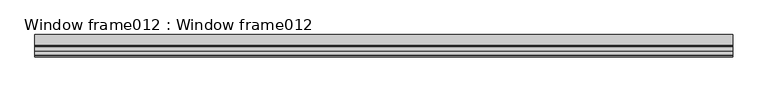
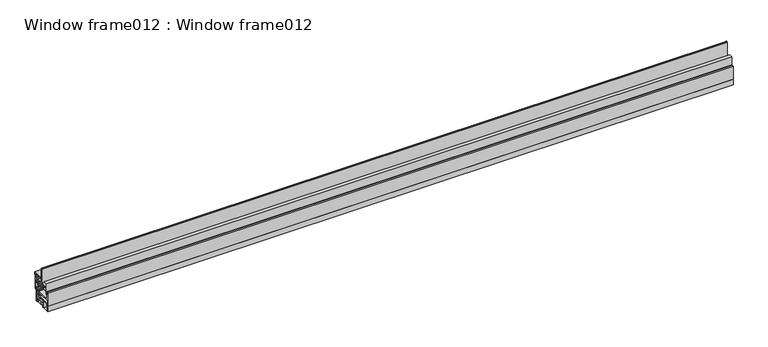
"""IFC4 building model written with IfcOpenShell, lengths in millimetres: proxy geometry, Window frame012 : Window frame012."""

from ifc_helpers import new_model, si_unit, frame, origin, place, context, project, spatial, polyline, outline, extrude, source, transform, mapped, element, save


def window_frame012_window_frame012_050a5667(model_context):
    return source(origin(), model_context, "Body", "SweptSolid", [
        extrude(outline(polyline([(-4639.5309365, 38938.6991655), (-4638.9555243, 38936.2575018), (-4636.7286164, 38936.2575018), (-4636.7286164, 38933.8445018), (-4638.9548305, 38933.8445018), (-4639.3785718, 38931.3856089), (-4640.7319367, 38931.3856089), (-4641.3675759, 38934.2475851), (-4641.3675759, 38936.108948), (-4640.7050488, 38938.6991655), (-4639.5309365, 38938.6991655)])), frame((12383.0178845, 0.0, 0.0), z_axis=(1.0, 0.0, 0.0), x_axis=(0.0, 1.0, 0.0)), (0.0, 0.0, 1.0), 2000.0),
        extrude(outline(polyline([(-4669.1560964, 38931.9215517), (-4669.7315086, 38934.3632154), (-4671.9584164, 38934.3632154), (-4671.9584164, 38936.7762154), (-4669.7322024, 38936.7762154), (-4669.3084611, 38939.2351083), (-4667.9550962, 38939.2351083), (-4667.319457, 38936.3731321), (-4667.319457, 38934.5117692), (-4667.9819841, 38931.9215517), (-4669.1560964, 38931.9215517)])), frame((12383.0178845, 0.0, 0.0), z_axis=(1.0, 0.0, 0.0), x_axis=(0.0, 1.0, 0.0)), (0.0, 0.0, 1.0), 2000.0),
        extrude(outline(polyline([(-4686.0427164, 38989.4601156), (-4686.0427164, 38981.9427334), (-4686.8742969, 38981.9427334), (-4686.8742969, 38985.318069), (-4690.1702164, 38985.318069), (-4690.1702164, 38986.511869), (-4686.8742969, 38986.511869), (-4686.8742969, 38989.4601156), (-4686.0427164, 38989.4601156)])), frame((12383.0178845, 0.0, 0.0), z_axis=(1.0, 0.0, 0.0), x_axis=(0.0, 1.0, 0.0)), (0.0, 0.0, 1.0), 2000.0),
        extrude(outline(polyline([(-4634.8744164, 38965.9106847), (-4634.8744164, 38973.4280669), (-4634.042836, 38973.4280669), (-4634.042836, 38970.0527312), (-4630.7469164, 38970.0527312), (-4630.7469164, 38968.8589312), (-4634.042836, 38968.8589312), (-4634.042836, 38965.9106847), (-4634.8744164, 38965.9106847)])), frame((12383.0178845, 0.0, 0.0), z_axis=(1.0, 0.0, 0.0), x_axis=(0.0, 1.0, 0.0)), (0.0, 0.0, 1.0), 2000.0),
        extrude(outline(polyline([(-4639.3829164, 39014.9345312), (-4628.8927164, 39014.9345312), (-4628.8927164, 38965.8617312), (-4633.2869164, 38965.8617312), (-4633.2869164, 38968.1229261), (-4632.0169164, 38968.1229261), (-4632.0169164, 38967.1317312), (-4630.7469164, 38967.1317312), (-4630.7469164, 38972.2117312), (-4632.0258979, 38972.2117312), (-4632.0258979, 38971.3233198), (-4633.2869164, 38971.3233198), (-4633.2869164, 38988.1375312), (-4636.3613739, 38988.1375312), (-4636.3613739, 38990.1695312), (-4634.7347164, 38990.1695312), (-4634.7347164, 38991.9744739), (-4633.3123168, 38991.9744739), (-4633.3123168, 38990.1695312), (-4630.9247164, 38990.1695312), (-4630.9247164, 38999.6752218), (-4633.3117065, 38999.6752218), (-4633.3117065, 38997.6552203), (-4634.7347164, 38997.6552203), (-4634.7347164, 39001.7519312), (-4630.9247164, 39001.7519312), (-4630.9247164, 39012.9025312), (-4639.3829164, 39012.9025312), (-4639.3829164, 39014.9345312)])), frame((12383.0178845, 0.0, 0.0), z_axis=(1.0, 0.0, 0.0), x_axis=(0.0, 1.0, 0.0)), (0.0, 0.0, 1.0), 2000.0),
        extrude(outline(polyline([(-4649.4159164, 38951.9679312), (-4649.4159164, 38953.7713312), (-4689.9924164, 38953.7713312), (-4689.9924164, 38951.7401776), (-4688.5748922, 38948.9453312), (-4692.0244164, 38948.9453312), (-4692.0244164, 38989.6615312), (-4687.6302164, 38989.6615312), (-4687.6302164, 38987.3917784), (-4688.9241561, 38987.3917784), (-4688.9241561, 38988.3887876), (-4690.1702164, 38988.3887876), (-4690.1702164, 38983.3249754), (-4688.9233832, 38983.3249754), (-4688.9233832, 38984.231851), (-4687.6302164, 38984.231851), (-4687.6302164, 38967.3857312), (-4647.0664164, 38967.3857312), (-4647.0664164, 38964.1085142), (-4648.3200073, 38964.1085142), (-4648.3200073, 38965.3537312), (-4650.8764164, 38965.3537312), (-4650.8764164, 38955.8033277), (-4646.287204, 38955.8033277), (-4646.287204, 38953.7713312), (-4648.0150337, 38953.7713312), (-4648.0150337, 38950.5963312), (-4651.5876164, 38950.5963312), (-4651.5876164, 38951.9679312), (-4649.4159164, 38951.9679312)]), holes=[polyline([(-4689.4844164, 38964.2107312), (-4689.4844164, 38956.9463312), (-4652.9084164, 38956.9463312), (-4652.9084164, 38964.2107312), (-4689.4844164, 38964.2107312)])]), frame((12383.0178845, 0.0, 0.0), z_axis=(1.0, 0.0, 0.0), x_axis=(0.0, 1.0, 0.0)), (0.0, 0.0, 1.0), 2000.0),
        extrude(outline(polyline([(-4642.727462, 38944.1955312), (-4667.0435164, 38944.1955312), (-4667.0435164, 38951.9425312), (-4653.0000564, 38951.9226402), (-4653.0000564, 38950.0739491), (-4646.0866776, 38950.0739491), (-4646.0866776, 38953.7713312), (-4639.2686164, 38953.7713312), (-4639.2686164, 38950.4926946), (-4640.962162, 38950.4926946), (-4640.962162, 38945.7214228), (-4642.727462, 38944.1955312)])), frame((12383.0178845, 0.0, 0.0), z_axis=(1.0, 0.0, 0.0), x_axis=(0.0, 1.0, 0.0)), (0.0, 0.0, 1.0), 2000.0),
        extrude(outline(polyline([(14383.0178845, -4647.9427164), (14383.0178845, -4660.7189164), (12383.0178845, -4660.7189164), (12383.0178845, -4647.9427164), (14383.0178845, -4647.9427164)])), frame((0.0, 0.0, 38934.6705312), z_axis=(0.0, 0.0, 1.0), x_axis=(1.0, 0.0, 0.0)), (0.0, 0.0, 1.0), 9.525),
        extrude(outline(polyline([(-4636.9064164, 38967.3857312), (-4636.9064164, 38972.2117312), (-4634.8744164, 38972.2117312), (-4634.8744164, 38931.4955312), (-4639.2686164, 38931.4955312), (-4639.2686164, 38933.7494749), (-4638.0264587, 38933.7494749), (-4638.0264587, 38932.7655312), (-4636.7286164, 38932.7655312), (-4636.7286164, 38937.8455312), (-4638.0088043, 38937.8455312), (-4638.0088043, 38936.9821562), (-4639.2686164, 38936.9821562), (-4639.2686164, 38953.7713312), (-4641.5038161, 38953.7713312), (-4641.5038161, 38955.8033277), (-4636.9064164, 38955.8033277), (-4636.9064164, 38965.3537312), (-4639.4738693, 38965.3537312), (-4639.4738693, 38964.0949034), (-4640.6951408, 38964.0949034), (-4640.6951408, 38967.3857312), (-4636.9064164, 38967.3857312)])), frame((12383.0178845, 0.0, 0.0), z_axis=(1.0, 0.0, 0.0), x_axis=(0.0, 1.0, 0.0)), (0.0, 0.0, 1.0), 2000.0),
        extrude(outline(polyline([(-4642.3510612, 38999.7199312), (-4644.8947164, 38999.7199312), (-4644.8947164, 38990.1695312), (-4640.3055043, 38990.1695312), (-4640.3055043, 38988.1375312), (-4642.0574073, 38988.1375312), (-4642.0574073, 38984.9625312), (-4646.293591, 38984.9625312), (-4646.293591, 38986.3341312), (-4643.3560584, 38986.3341312), (-4643.3560584, 38988.1375312), (-4684.0107164, 38988.1375312), (-4684.0107164, 38985.877289), (-4682.6339998, 38983.3115312), (-4686.0427164, 38983.3115312), (-4686.0427164, 39014.9345312), (-4675.5525164, 39014.9345312), (-4675.5525164, 39012.9025312), (-4684.0107164, 39012.9025312), (-4684.0107164, 39001.7519312), (-4662.2175164, 39001.7519312), (-4662.2175164, 39045.282064), (-4660.6427164, 39045.282064), (-4660.6427164, 39014.954464), (-4660.6427173, 39001.7519316), (-4641.0847164, 39001.7519312), (-4641.0847164, 38997.6552203), (-4642.3510612, 38997.6552203), (-4642.3510612, 38999.7199312)]), holes=[polyline([(-4653.8842334, 38991.3125312), (-4646.9267164, 38991.3125312), (-4646.9267164, 38998.5769312), (-4650.5636291, 38998.5769312), (-4650.5636291, 38999.7199312), (-4660.3350067, 38999.7199312), (-4660.3350067, 38998.5769312), (-4666.0374507, 38998.5769312), (-4666.0374507, 38999.7199312), (-4675.6009273, 38999.7199312), (-4675.6009273, 38998.5769312), (-4679.5213594, 38998.5769312), (-4679.5213594, 38999.7199312), (-4683.5027164, 38999.7199312), (-4683.5027164, 38990.1695312), (-4679.4756188, 38990.1695312), (-4679.4756188, 38991.3125312), (-4670.5952491, 38991.3125312), (-4670.5952491, 38990.1695312), (-4666.1105117, 38990.1695312), (-4666.1105117, 38991.3125312), (-4662.2140522, 38991.3125312), (-4662.2140522, 38990.1695312), (-4653.8842334, 38990.1695312), (-4653.8842334, 38991.3125312)])]), frame((12383.0178845, 0.0, 0.0), z_axis=(1.0, 0.0, 0.0), x_axis=(0.0, 1.0, 0.0)), (0.0, 0.0, 1.0), 2000.0),
        extrude(outline(polyline([(-4692.0244164, 38931.4955312), (-4692.0244164, 38948.9453312), (-4688.5096075, 38948.9453312), (-4689.5028424, 38951.1888746), (-4688.0078306, 38952.6351179), (-4687.201703, 38952.6351179), (-4687.201703, 38947.5483312), (-4690.6274164, 38947.5483312), (-4690.6274164, 38932.8925312), (-4673.3554164, 38932.8925312), (-4673.3554164, 38953.3395312), (-4649.4159164, 38953.3395312), (-4649.4159164, 38951.9679312), (-4671.9584164, 38951.9425312), (-4671.9584164, 38939.1316542), (-4669.438631, 38939.1316542), (-4669.438631, 38936.9480375), (-4670.6122465, 38936.9480375), (-4670.6122465, 38937.8455312), (-4671.9584164, 38937.8455312), (-4671.9584164, 38932.775186), (-4670.6448459, 38932.775186), (-4670.6448459, 38933.7042936), (-4669.4060287, 38933.7042936), (-4669.4060287, 38931.4955312), (-4692.0244164, 38931.4955312)])), frame((12383.0178845, 0.0, 0.0), z_axis=(1.0, 0.0, 0.0), x_axis=(0.0, 1.0, 0.0)), (0.0, 0.0, 1.0), 2000.0),
        extrude(outline(polyline([(-4660.6427164, 39046.6845312), (-4659.6267164, 39046.6845312), (-4659.6267164, 39015.9505312), (-4627.8767164, 39015.9505312), (-4627.8767164, 39008.5845312), (-4628.8927164, 39008.5845312), (-4628.8927164, 39014.9345312), (-4660.6427164, 39014.9345312), (-4660.6427164, 39046.6845312)])), frame((12383.0178845, 0.0, 0.0), z_axis=(1.0, 0.0, 0.0), x_axis=(0.0, 1.0, 0.0)), (0.0, 0.0, 1.0), 2000.0),
    ])


if __name__ == "__main__":
    model = new_model("IFC4")
    model_context = context("Model", 3, world=origin())
    ifc_project = project(units=[si_unit("LENGTHUNIT", "METRE", prefix="MILLI")], contexts=[model_context])
    site = spatial("IfcSite", under=ifc_project)
    building = spatial("IfcBuilding", under=site)
    placement = place(None, origin())
    window_frame012_window_frame012_shape = window_frame012_window_frame012_050a5667(model_context)
    element("IfcBuildingElementProxy", 1, Name="Window frame012 : Window frame012", ObjectType="Window frame012 : Window frame012", at=placement, inside=building, context=model_context, shape_type="MappedRepresentation", body=[
        mapped(window_frame012_window_frame012_shape, transform((0.0, 0.0, 0.0), x_axis=(1.0, 0.0, 0.0), y_axis=(0.0, 1.0, 0.0), z_axis=(0.0, 0.0, 1.0))),
    ])
    save(model, "model.ifc")

# Revit data of these elements
# Type "Window frame012 : Window frame012"
#   NameOverride = "Window frame012"
# Element 1 (IfcBuildingElementProxy, "Window frame012 : Window frame012")
#   Materials on its faces: "FLEETWOOD SERIES 250-T-01 CASEMENT WINDOW FRAME"
# Materials
#   "FLEETWOOD SERIES 250-T-01 CASEMENT WINDOW FRAME": class "Unassigned", colour RGB 128 128 128, transparency 0
